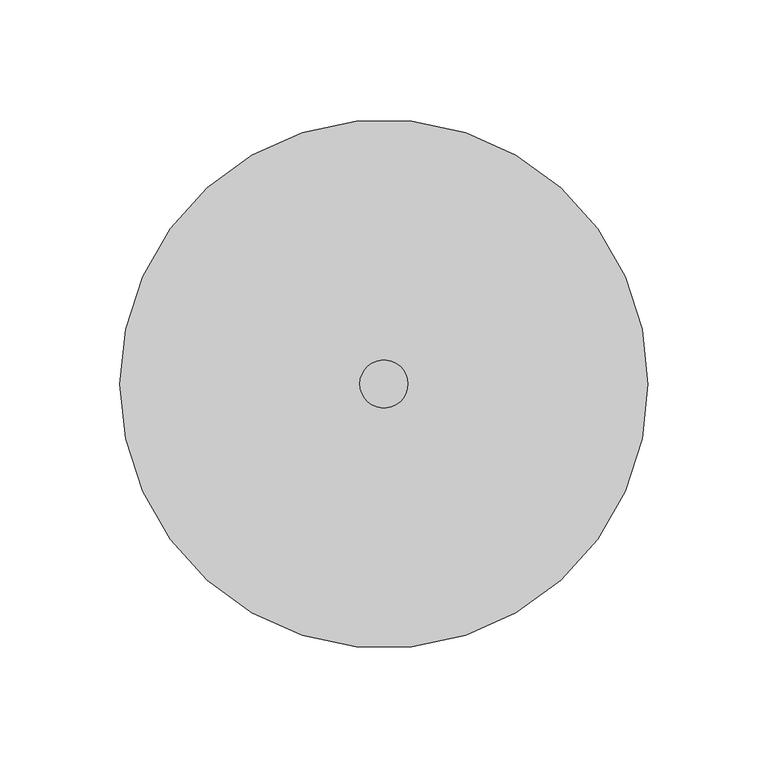
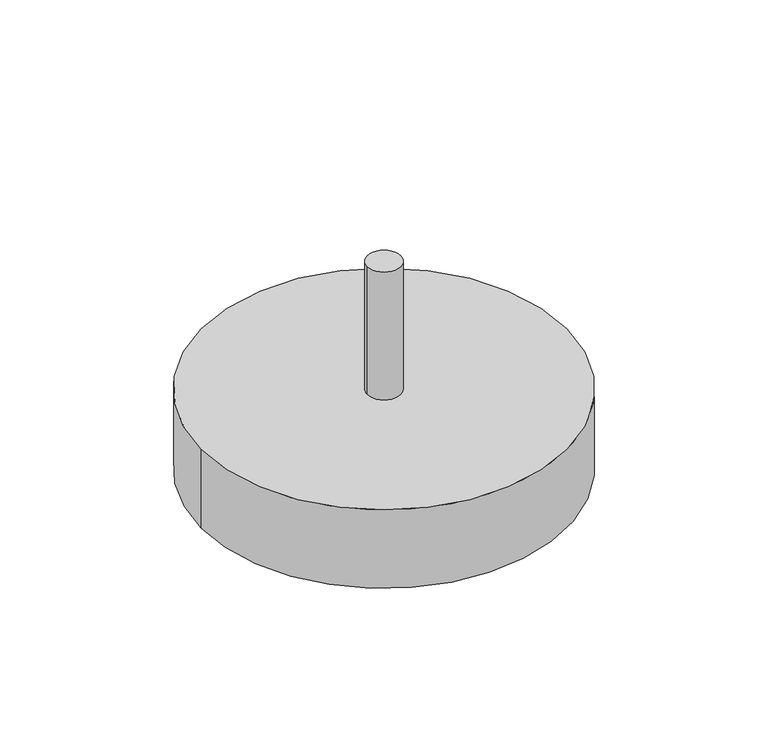
"""IFC4 building model written with IfcOpenShell, lengths in millimetres: electric appliance geometry, Wifi Access Point : Wifi Access Point."""

from ifc_helpers import new_model, si_unit, point, frame, origin, origin_with_axes, origin_2d, place, context, project, spatial, circle_curve, trimmed, segment, composite_curve, outline, extrude, source, transform, mapped, element, save


def electric_appliance_a5c8b711(model_context):
    return source(origin(), model_context, "Body", "SweptSolid", [
        extrude(outline(composite_curve([segment(trimmed(circle_curve(origin_2d(), 10.0), [point((-10.0, 0.0))], [point((10.0, 0.0))], False, "CARTESIAN"), True, "CONTINUOUS"), segment(trimmed(circle_curve(origin_2d(), 10.0), [point((10.0, 0.0))], [point((-10.0, 0.0))], False, "CARTESIAN"), True, "CONTINUOUS")], self_intersect=False)), frame((0.0, 0.0, 50.0), z_axis=(0.0, 0.0, 1.0), x_axis=(1.0, 0.0, 0.0)), (0.0, 0.0, 1.0), 81.4052538),
        extrude(outline(composite_curve([segment(trimmed(circle_curve(origin_2d(), 110.0), [point((-110.0, 0.0))], [point((110.0, 0.0))], False, "CARTESIAN"), True, "CONTINUOUS"), segment(trimmed(circle_curve(origin_2d(), 110.0), [point((110.0, 0.0))], [point((-110.0, 0.0))], False, "CARTESIAN"), True, "CONTINUOUS")], self_intersect=False)), origin_with_axes(), (0.0, 0.0, 1.0), 50.0),
    ])


if __name__ == "__main__":
    model = new_model("IFC4")
    model_context = context("Model", 3, world=origin())
    ifc_project = project(units=[si_unit("LENGTHUNIT", "METRE", prefix="MILLI")], contexts=[model_context])
    site = spatial("IfcSite", under=ifc_project)
    building = spatial("IfcBuilding", under=site)
    placement = place(None, origin())
    electric_appliance_shape = electric_appliance_a5c8b711(model_context)
    element("IfcElectricAppliance", 1, ObjectType="Wifi Access Point : Wifi Access Point", at=placement, inside=building, context=model_context, shape_type="MappedRepresentation", body=[
        mapped(electric_appliance_shape, transform((0.0, 0.0, 0.0), x_axis=(1.0, 0.0, 0.0), y_axis=(0.0, 1.0, 0.0), z_axis=(0.0, 0.0, 1.0))),
    ])
    save(model, "model.ifc")

# Revit data of these elements
# Type "Wifi Access Point : Wifi Access Point"
#   Default Elevation = 1.2 m
